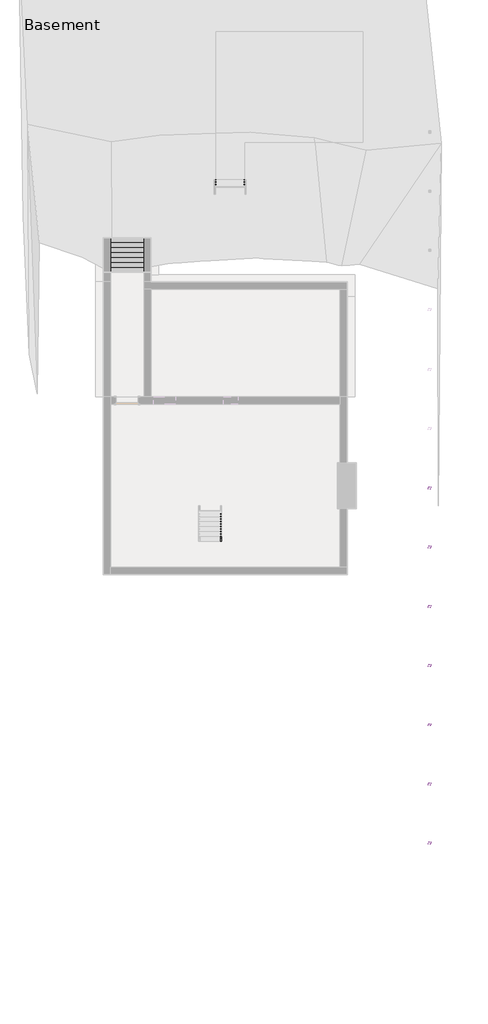
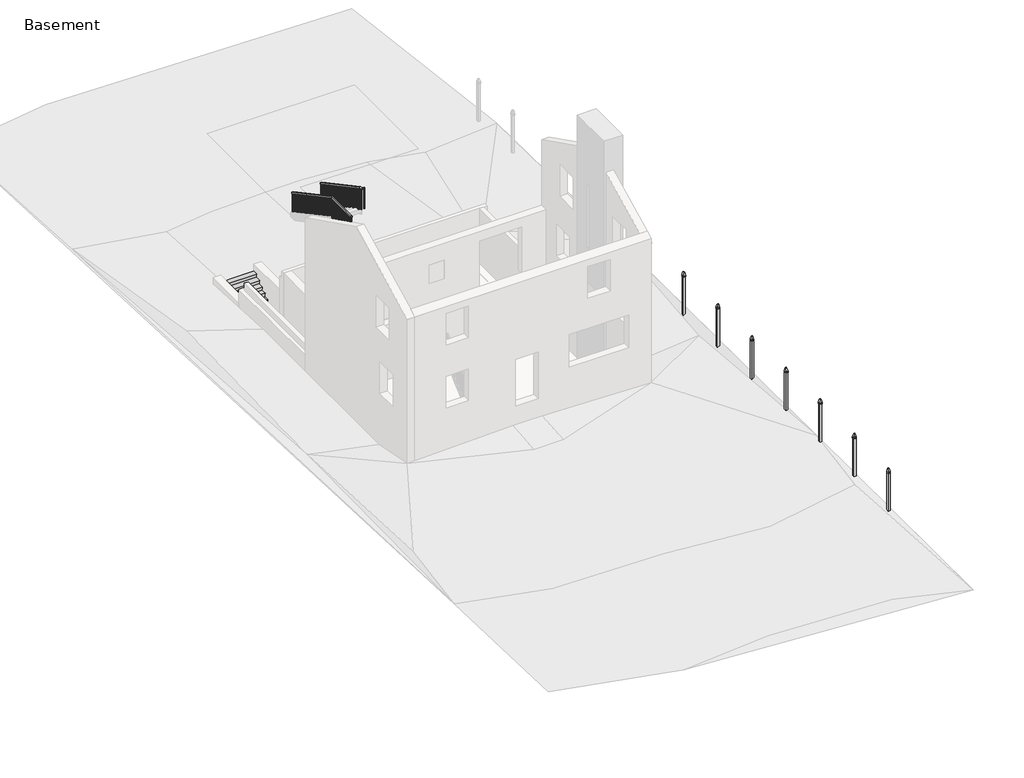
# One storey, part 2 of 3: 7 proxies, 3 railings, 1 stair flight.
# Revit data of these elements (continued)
# Type "SUP_Post : 4\" x 4\""
#   W = 0' - 3 1/2"
#   Post Offset = 0' - 2 1/2"
#   Bottom Extension = 0' - 9"
#   built-in parameter 1152166 = 4.75 (stored number, unit not read)
#   built-in parameter 1152165 [instance default] = 0.25 (stored number, unit not read)
#   D = 0' - 3 1/2"
#   Support Material = Pine
# Type "Handrail - Rectangular"
#   Assembly Code = "C2010400"
#   built-in parameter 1008612 = 0.0416667 (stored number, unit not read)
#   built-in parameter 1008611 = 0.0416667 (stored number, unit not read)
#   built-in parameter 1008609 = 0.333333 (stored number, unit not read)
#   built-in parameter 1008604 = 0.166667 (stored number, unit not read)
#   built-in parameter 1008603 = 0.166667 (stored number, unit not read)
#   Railing Height = 3' - 0"
#   built-in parameter 1008630 = 2
#   built-in parameter 1008610 = 2
#   built-in parameter 1008618 = Baluster - Square : 3/4"
# Elements 1, 2, 3, 4, 5, 6, 7 (IfcBuildingElementProxy, "SUP_Post : 4\" x 4\"")
#   built-in parameter 1152165 = 0.208333 (stored number, unit not read)
#   Materials on its faces: "Pine"
# Element 8 (IfcRailing, "Handrail - Rectangular")
#   Phase Created = Existing
#   Materials on its faces: "Maple - Semigloss(Rotated)"
# Elements 9, 10 (IfcRailing, "Handrail - Rectangular")
#   Phase Created = New Construction
#   Materials on its faces: "Maple - Semigloss(Rotated)"
# Element 11 (IfcStairFlight, "3/4\" Nosing")
#   Phase Created = New Construction
#   Materials on its faces: "Concrete, Cast-in-Place gray"
# Materials
#   "Pine": class "Wood", colour RGB 229 189 132, transparency 0, Description = "Pinus Echinata", Cost = 0
#   "Maple - Semigloss(Rotated)": class "Wood", colour RGB 196 161 118, transparency 0, Description = "Acer Saccharum", Cost = 0
#   "Concrete, Cast-in-Place gray": class "Concrete", colour RGB 192 192 192, transparency 0, Description = "Cast-in-place concrete", Cost = 0
